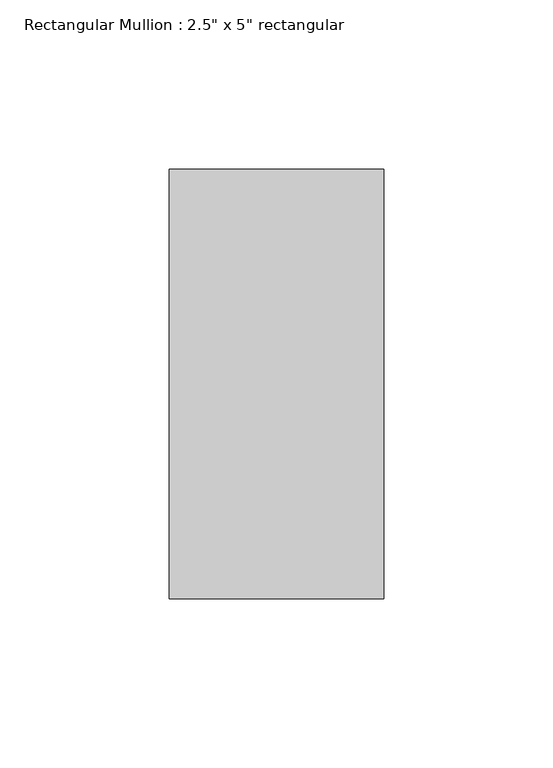
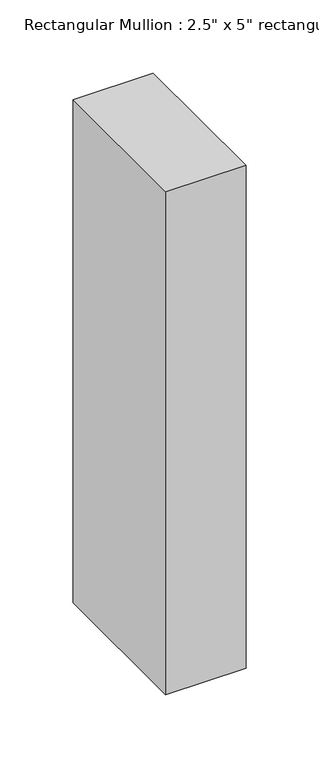
"""IFC4 building model written with IfcOpenShell, lengths in millimetres: member geometry."""

from ifc_helpers import new_model, si_unit, frame, origin, place, context, project, spatial, polyline, outline, extrude, source, transform, mapped, element, save


def member_9d079ec4(model_context):
    return source(origin(), model_context, "Body", "SweptSolid", [
        extrude(outline(polyline([(0.0, 63.5), (0.0, -63.5), (-63.5, -63.5), (-63.5, 63.5), (0.0, 63.5)])), frame((0.0, 0.0, -420.214047), z_axis=(0.0, 0.0, 1.0), x_axis=(1.0, 0.0, 0.0)), (0.0, 0.0, 1.0), 420.214047),
    ])


if __name__ == "__main__":
    model = new_model("IFC4")
    model_context = context("Model", 3, world=origin())
    ifc_project = project(units=[si_unit("LENGTHUNIT", "METRE", prefix="MILLI")], contexts=[model_context])
    site = spatial("IfcSite", under=ifc_project)
    building = spatial("IfcBuilding", under=site)
    placement = place(None, origin())
    member_shape = member_9d079ec4(model_context)
    element("IfcMember", 1, ObjectType="Rectangular Mullion : 2.5\" x 5\" rectangular", at=placement, inside=building, context=model_context, shape_type="MappedRepresentation", body=[
        mapped(member_shape, transform((0.0, 0.0, 0.0), x_axis=(1.0, 0.0, 0.0), y_axis=(0.0, 1.0, 0.0), z_axis=(0.0, 0.0, 1.0))),
    ])
    save(model, "model.ifc")

# Revit data of these elements
# Type "Rectangular Mullion : 2.5\" x 5\" rectangular"
#   built-in parameter 1007304 = 0.416667 (stored number, unit not read)
#   built-in parameter 1007301 = 0.104167 (stored number, unit not read)
#   built-in parameter 1007300 = 0.104167 (stored number, unit not read)
# Element 1 (IfcMember, "Rectangular Mullion : 2.5\" x 5\" rectangular")
#   Materials on its faces: "Metal - Aluminum 2"
# Materials
#   "Metal - Aluminum 2": class "Metal", colour RGB 189 187 185, transparency 0
